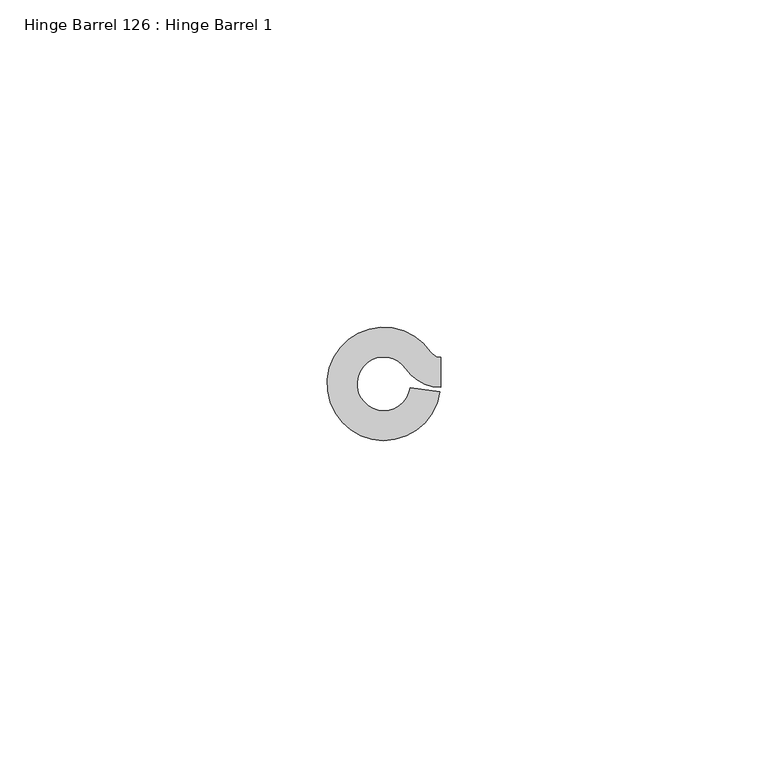
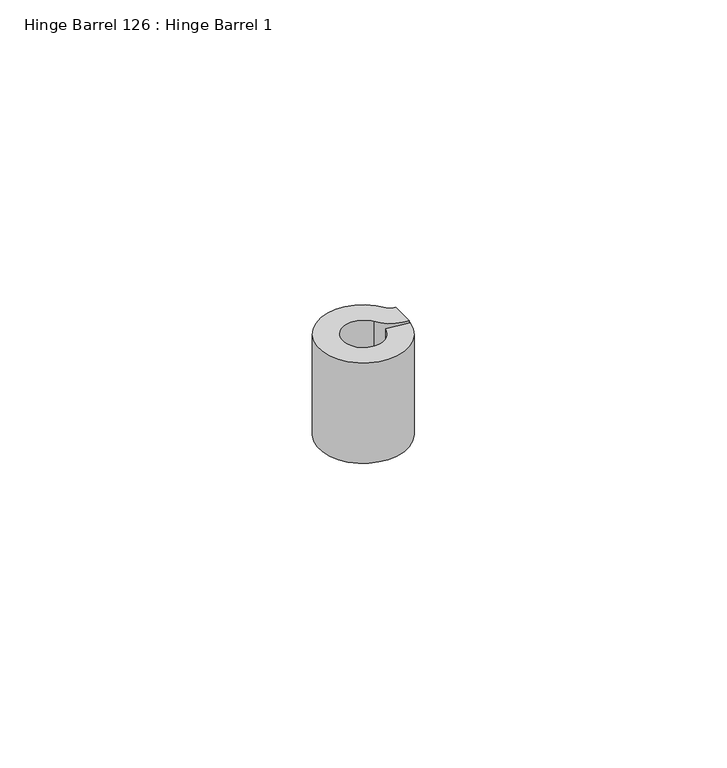
"""IFC4 building model written with IfcOpenShell, lengths in millimetres: proxy geometry, Hinge Barrel 126 : Hinge Barrel 1."""

from ifc_helpers import new_model, si_unit, point, frame, frame_2d, origin, place, context, project, spatial, polyline, circle_curve, trimmed, segment, composite_curve, outline, extrude, source, transform, mapped, element, save


def hinge_barrel_126_hinge_barrel_1_73cfb3f3(model_context):
    return source(origin(), model_context, "Body", "SweptSolid", [
        extrude(outline(composite_curve([segment(trimmed(circle_curve(frame_2d((587319.1320739, -534100.7049841)), 4.0894), [point((587322.5194669, -534098.4139665))], [point((587323.1821338, -534101.2708529))], True, "CARTESIAN"), True, "CONTINUOUS"), segment(polyline([(587323.1821338, -534101.2708529), (587327.7022899, -534101.9024028)]), True, "CONTINUOUS"), segment(trimmed(circle_curve(frame_2d((587319.1320739, -534100.7049841)), 8.6534625), [point((587327.7022899, -534101.9024028))], [point((587326.3000393, -534095.8570273))], False, "CARTESIAN"), True, "CONTINUOUS"), segment(trimmed(circle_curve(frame_2d((587327.8245257, -534094.8259615)), 1.8404226), [point((587326.3000393, -534095.8570273))], [point((587327.8245257, -534096.6663841))], True, "CARTESIAN"), True, "CONTINUOUS"), segment(polyline([(587327.8245257, -534096.6663841), (587327.8245257, -534101.2304466)]), True, "CONTINUOUS"), segment(trimmed(circle_curve(frame_2d((587327.8245257, -534094.8259615)), 6.4044851), [point((587327.8245257, -534101.2304466))], [point((587322.5194669, -534098.4139665))], False, "CARTESIAN"), True, "CONTINUOUS")], self_intersect=False)), frame((0.0, 0.0, 1250.95), z_axis=(0.0, 0.0, 1.0), x_axis=(1.0, 0.0, 0.0)), (0.0, 0.0, 1.0), 20.8359375),
    ])


if __name__ == "__main__":
    model = new_model("IFC4")
    model_context = context("Model", 3, world=origin())
    ifc_project = project(units=[si_unit("LENGTHUNIT", "METRE", prefix="MILLI")], contexts=[model_context])
    site = spatial("IfcSite", under=ifc_project)
    building = spatial("IfcBuilding", under=site)
    placement = place(None, origin())
    hinge_barrel_126_hinge_barrel_1_shape = hinge_barrel_126_hinge_barrel_1_73cfb3f3(model_context)
    element("IfcBuildingElementProxy", 1, Name="Hinge Barrel 126 : Hinge Barrel 1", ObjectType="Hinge Barrel 126 : Hinge Barrel 1", at=placement, inside=building, context=model_context, shape_type="MappedRepresentation", body=[
        mapped(hinge_barrel_126_hinge_barrel_1_shape, transform((0.0, 0.0, 0.0), x_axis=(1.0, 0.0, 0.0), y_axis=(0.0, 1.0, 0.0), z_axis=(0.0, 0.0, 1.0))),
    ])
    save(model, "model.ifc")

# Revit data of these elements
# Element 1 (IfcBuildingElementProxy, "Hinge Barrel 126 : Hinge Barrel 1")
#   Materials on its faces: "6\"X6\" WELD-ON STL BUTT HINGE"
# Materials
#   "6\"X6\" WELD-ON STL BUTT HINGE": class "Metal", colour RGB 189 187 185, transparency 0, Description = "Carbon steel", Cost = 0
